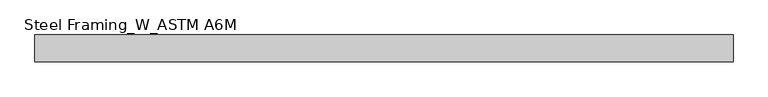
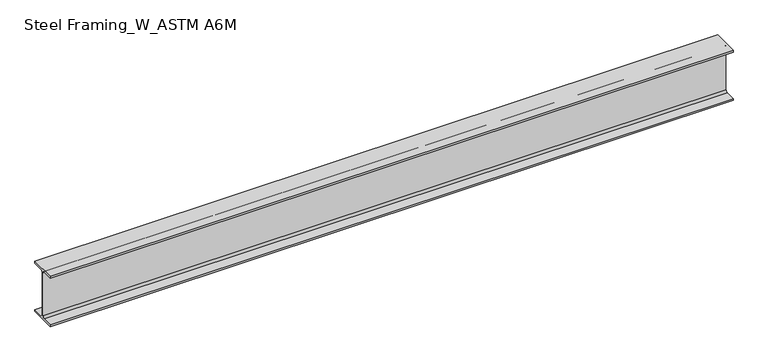
"""IFC4 building model written with IfcOpenShell, lengths in millimetres: beam geometry, Steel Framing_W_ASTM A6M : H_SB_AR_S02_W200x22.5_J1."""

import ifcopenshell
import ifcopenshell.guid

model = None  # the IFC model being written
_history = None  # IfcOwnerHistory: only IFC2X3 demands one
_inside = {}  # id of a spatial element -> (the spatial element, [elements in it])
_under = {}  # id of a project, library or spatial element -> (it, [spatial elements below it])
_declared = {}  # id of a project -> (the project, [libraries it declares])
_typed = {}  # id of a type object -> (the type object, [elements of that type])
_made_of = {}  # id of a material, layer set ... -> (it, [elements and type objects made of it])


def new_model(schema):
    """Start an empty IFC model of exactly this schema.

    Asked for "IFC4X3", IfcOpenShell would pick the latest addendum, in which some entities
    have other attributes; the version numbers below select the first issue.
    IFC2X3 requires an IfcOwnerHistory on every rooted entity: one is made here for all.
    """
    global model, _history
    if schema == "IFC4X3":
        model = ifcopenshell.file(schema_version=(4, 3, 0, 0))
    else:
        model = ifcopenshell.file(schema=schema)
    _inside.clear()
    _under.clear()
    _declared.clear()
    _typed.clear()
    _made_of.clear()
    _history = None
    if model.schema == "IFC2X3":
        org = make("IfcOrganization", Name="unknown")
        user = make(
            "IfcPersonAndOrganization",
            ThePerson=make("IfcPerson", FamilyName="unknown"),
            TheOrganization=org,
        )
        app = make(
            "IfcApplication",
            ApplicationDeveloper=org,
            Version="unknown",
            ApplicationFullName="unknown",
            ApplicationIdentifier="unknown",
        )
        _history = make(
            "IfcOwnerHistory",
            OwningUser=user,
            OwningApplication=app,
            ChangeAction="ADDED",
            CreationDate=0,
        )
    return model


def make(cls, **values):
    """One entity of the class cls with the attributes given. An attribute that is None is left unset."""
    return model.create_entity(
        cls, **{name: value for name, value in values.items() if value is not None}
    )


def rooted(cls, **values):
    """An entity with a GlobalId (a new one), such as an element, a storey or a relation."""
    return make(cls, GlobalId=ifcopenshell.guid.new(), OwnerHistory=_history, **values)


def si_unit(unit_type, name, prefix=None):
    """IfcSIUnit, for example si_unit("LENGTHUNIT", "METRE", prefix="MILLI")."""
    return make("IfcSIUnit", UnitType=unit_type, Prefix=prefix, Name=name)


def assignment(units):
    """IfcUnitAssignment: the units of a project."""
    return None if units is None else make("IfcUnitAssignment", Units=units)


def point(xyz):
    """IfcCartesianPoint."""
    return None if xyz is None else make("IfcCartesianPoint", Coordinates=xyz)


def direction(xyz):
    """IfcDirection."""
    return None if xyz is None else make("IfcDirection", DirectionRatios=xyz)


def frame(location, z_axis=None, x_axis=None):
    """IfcAxis2Placement3D, a coordinate frame: its origin and axes. An axis left out is left unset."""
    return make(
        "IfcAxis2Placement3D",
        Location=point(location),
        Axis=direction(z_axis),
        RefDirection=direction(x_axis),
    )


def frame_2d(location, x_axis=None):
    """IfcAxis2Placement2D, a coordinate frame in the plane: its origin and x axis."""
    return make(
        "IfcAxis2Placement2D", Location=point(location), RefDirection=direction(x_axis)
    )


def origin():
    """The frame at (0, 0, 0) with its axes left unset."""
    return frame((0.0, 0.0, 0.0))


def place(relative_to, where):
    """IfcLocalPlacement: puts the frame where relative to a parent placement (None: the world)."""
    return make(
        "IfcLocalPlacement", PlacementRelTo=relative_to, RelativePlacement=where
    )


def context(
    kind, dimensions, precision=None, world=None, true_north=None, identifier=None
):
    """IfcGeometricRepresentationContext, for example the 3D "Model" context."""
    return make(
        "IfcGeometricRepresentationContext",
        ContextIdentifier=identifier,
        ContextType=kind,
        CoordinateSpaceDimension=dimensions,
        Precision=precision,
        WorldCoordinateSystem=world,
        TrueNorth=true_north,
    )


def project(units=None, contexts=None):
    """IfcProject with its units and contexts."""
    return rooted(
        "IfcProject",
        Name="project",
        RepresentationContexts=contexts,
        UnitsInContext=assignment(units),
    )


def spatial(cls, under=None, at=None, **own):
    """A site, building, storey or space (cls), placed at a placement, below another one or the project."""
    s = rooted(cls, ObjectPlacement=at, **own)
    if under is not None:
        _under.setdefault(under.id(), (under, []))[1].append(s)
    return s


def polyline(points):
    """IfcPolyline through the points."""
    return make("IfcPolyline", Points=[point(p) for p in points])


def circle_curve(where, radius):
    """IfcCircle in the frame where."""
    return make("IfcCircle", Position=where, Radius=radius)


def trimmed(basis, trim1, trim2, sense, master):
    """IfcTrimmedCurve: the piece of a basis curve between two trims."""
    return make(
        "IfcTrimmedCurve",
        BasisCurve=basis,
        Trim1=trim1,
        Trim2=trim2,
        SenseAgreement=sense,
        MasterRepresentation=master,
    )


def segment(curve, same_sense, transition):
    """IfcCompositeCurveSegment."""
    return make(
        "IfcCompositeCurveSegment",
        Transition=transition,
        SameSense=same_sense,
        ParentCurve=curve,
    )


def composite_curve(segments, self_intersect=None):
    """IfcCompositeCurve: segments joined end to end."""
    return make("IfcCompositeCurve", Segments=segments, SelfIntersect=self_intersect)


def outline(outer, holes=None, kind="AREA"):
    """IfcArbitraryClosedProfileDef: a profile drawn as a closed curve; with holes, ...WithVoids."""
    if holes is None:
        return make("IfcArbitraryClosedProfileDef", ProfileType=kind, OuterCurve=outer)
    return make(
        "IfcArbitraryProfileDefWithVoids",
        ProfileType=kind,
        OuterCurve=outer,
        InnerCurves=holes,
    )


def extrude(swept, where, along, depth):
    """IfcExtrudedAreaSolid: the profile swept, set in the frame where, extruded along a direction by depth."""
    return make(
        "IfcExtrudedAreaSolid",
        SweptArea=swept,
        Position=where,
        ExtrudedDirection=direction(along),
        Depth=depth,
    )


def shape(context_of_items, identifier, shape_type, items):
    """IfcShapeRepresentation: the items that make up one representation, for example the "Body"."""
    return make(
        "IfcShapeRepresentation",
        ContextOfItems=context_of_items,
        RepresentationIdentifier=identifier,
        RepresentationType=shape_type,
        Items=items,
    )


def source(mapping_origin, context_of_items, identifier, shape_type, items):
    """IfcRepresentationMap: a shape defined once, which mapped items show again and again."""
    return make(
        "IfcRepresentationMap",
        MappingOrigin=mapping_origin,
        MappedRepresentation=shape(context_of_items, identifier, shape_type, items),
    )


def transform(
    local_origin,
    x_axis=None,
    y_axis=None,
    z_axis=None,
    scale=None,
    scale2=None,
    scale3=None,
    uniform=True,
):
    """IfcCartesianTransformationOperator3D, or its non-uniform kind. x_axis, y_axis, z_axis: its Axis1, 2, 3."""
    if uniform:
        return make(
            "IfcCartesianTransformationOperator3D",
            Axis1=direction(x_axis),
            Axis2=direction(y_axis),
            LocalOrigin=point(local_origin),
            Scale=scale,
            Axis3=direction(z_axis),
        )
    return make(
        "IfcCartesianTransformationOperator3DnonUniform",
        Axis1=direction(x_axis),
        Axis2=direction(y_axis),
        LocalOrigin=point(local_origin),
        Scale=scale,
        Axis3=direction(z_axis),
        Scale2=scale2,
        Scale3=scale3,
    )


def mapped(mapping_source, mapping_target):
    """IfcMappedItem: shows the shape of a source again, moved by a transform."""
    return make(
        "IfcMappedItem", MappingSource=mapping_source, MappingTarget=mapping_target
    )


def made_of(thing, what):
    """Note that an element or type object is made of a material, layer set ...; save() writes the relation."""
    if what is not None:
        _made_of.setdefault(what.id(), (what, []))[1].append(thing)
    return thing


def element(
    cls,
    number,
    at=None,
    inside=None,
    cuts=None,
    type_object=None,
    material=None,
    context=None,
    identifier="Body",
    shape_type=None,
    held_by="IfcProductDefinitionShape",
    body=None,
    shapes=None,
    **own,
):
    """One element of the class cls, such as IfcWall. Its Tag is "e" and its number.

    at: its placement. inside: the storey or other place that contains it. cuts: it is an
    opening in that element (IfcRelVoidsElement). A single representation is given by context,
    identifier, shape_type and body (its items); several are given by shapes. held_by: the class
    of the entity that holds the representations. save() writes the other relations.
    """
    e = rooted(cls, Tag="e%d" % number, ObjectPlacement=at, **own)
    if body is not None:
        shapes = [shape(context, identifier, shape_type, body)]
    if shapes is not None:
        e.Representation = make(held_by, Representations=shapes)
    if inside is not None:
        _inside.setdefault(inside.id(), (inside, []))[1].append(e)
    if cuts is not None:
        rooted(
            "IfcRelVoidsElement", RelatingBuildingElement=cuts, RelatedOpeningElement=e
        )
    if type_object is not None:
        _typed.setdefault(type_object.id(), (type_object, []))[1].append(e)
    return made_of(e, material)


def aggregate(whole, parts):
    """IfcRelAggregates: a whole, such as a stair, and the parts it consists of."""
    return rooted("IfcRelAggregates", RelatingObject=whole, RelatedObjects=parts)


def save(model, path):
    """Write the relations noted so far, then the file.

    IfcRelAggregates (storeys below a building ...), IfcRelContainedInSpatialStructure (elements
    in a storey), IfcRelDefinesByType, IfcRelAssociatesMaterial and IfcRelDeclares: one each for
    every whole, place, type object, material and project.
    """
    for whole, parts in _under.values():
        aggregate(whole, parts)
    for where, things in _inside.values():
        rooted(
            "IfcRelContainedInSpatialStructure",
            RelatedElements=things,
            RelatingStructure=where,
        )
    for kind, things in _typed.values():
        rooted("IfcRelDefinesByType", RelatedObjects=things, RelatingType=kind)
    for what, things in _made_of.values():
        rooted("IfcRelAssociatesMaterial", RelatedObjects=things, RelatingMaterial=what)
    for by, libraries in _declared.values():
        rooted("IfcRelDeclares", RelatingContext=by, RelatedDefinitions=libraries)
    model.write(path)


def steel_framing_w_astm_a6m_d2b621d1(model_context):
    return source(origin(), model_context, "Body", "SweptSolid", [
        extrude(outline(composite_curve([segment(polyline([(51.0, -95.0), (51.0, -103.0), (-51.0, -103.0), (-51.0, -95.0), (-10.71, -95.0)]), True, "CONTINUOUS"), segment(trimmed(circle_curve(frame_2d((-10.71, -87.4)), 7.6), [point((-10.71, -95.0))], [point((-3.11, -87.4))], True, "CARTESIAN"), True, "CONTINUOUS"), segment(polyline([(-3.11, -87.4), (-3.11, 87.4)]), True, "CONTINUOUS"), segment(trimmed(circle_curve(frame_2d((-10.71, 87.4)), 7.6), [point((-3.11, 87.4))], [point((-10.71, 95.0))], True, "CARTESIAN"), True, "CONTINUOUS"), segment(polyline([(-10.71, 95.0), (-51.0, 95.0), (-51.0, 103.0), (51.0, 103.0), (51.0, 95.0), (10.71, 95.0)]), True, "CONTINUOUS"), segment(trimmed(circle_curve(frame_2d((10.71, 87.4)), 7.6), [point((10.71, 95.0))], [point((3.11, 87.4))], True, "CARTESIAN"), True, "CONTINUOUS"), segment(polyline([(3.11, 87.4), (3.11, -87.4)]), True, "CONTINUOUS"), segment(trimmed(circle_curve(frame_2d((10.71, -87.4)), 7.6), [point((3.11, -87.4))], [point((10.71, -95.0))], True, "CARTESIAN"), True, "CONTINUOUS"), segment(polyline([(10.71, -95.0), (51.0, -95.0)]), True, "CONTINUOUS")], self_intersect=False)), frame((-1319.7, 0.0, 0.0), z_axis=(1.0, 0.0, 0.0), x_axis=(0.0, 1.0, 0.0)), (0.0, 0.0, 1.0), 2639.4),
    ])


if __name__ == "__main__":
    model = new_model("IFC4")
    model_context = context("Model", 3, world=origin())
    ifc_project = project(units=[si_unit("LENGTHUNIT", "METRE", prefix="MILLI")], contexts=[model_context])
    site = spatial("IfcSite", under=ifc_project)
    building = spatial("IfcBuilding", under=site)
    placement = place(None, origin())
    steel_framing_w_astm_a6m_shape = steel_framing_w_astm_a6m_d2b621d1(model_context)
    element("IfcBeam", 1, ObjectType="Steel Framing_W_ASTM A6M : H_SB_AR_S02_W200x22.5_J1", at=placement, inside=building, context=model_context, shape_type="MappedRepresentation", body=[
        mapped(steel_framing_w_astm_a6m_shape, transform((0.0, 0.0, 0.0), x_axis=(1.0, 0.0, 0.0), y_axis=(0.0, 1.0, 0.0), z_axis=(0.0, 0.0, 1.0))),
    ])
    save(model, "model.ifc")

# Revit data of these elements
# Type "Steel Framing_W_ASTM A6M : H_SB_AR_S02_W200x22.5_J1"
#   Section Name Key = "W8x15"
#   Width = 10.2 cm
#   Web Thickness = 0.622 cm
#   Web Fillet = 0.76 cm
#   Warping Constant = 13900.0 cm⁶
#   Torsional Moment of Inertia = 5.70 cm⁴
#   Section Area = 28.6 cm²
#   Plastic Modulus weak axis = 43.8 cm³
#   Plastic Modulus strong axis = 223.0 cm³
#   Perimeter = 0.795 m²/m
#   Nominal Weight = 22.50 kgf/m
#   Moment of Inertia weak axis = 142.00 cm⁴
#   Moment of Inertia strong axis = 2000.00 cm⁴
#   Height = 20.6 cm
#   Flange Thickness = 0.8 cm
#   Elastic Modulus weak axis = 27.9 cm³
#   Elastic Modulus strong axis = 193.0 cm³
#   Centroid Vertical = 10.3 cm
#   Centroid Horizontal = 5.1 cm
#   Length [instance default] = 1500 mm
#   Structural Material [instance default] = Steel, 45-345
#   Bolt Spacing = 0
#   Assembly Code = ""
# Element 1 (IfcBeam, "Steel Framing_W_ASTM A6M : H_SB_AR_S02_W200x22.5_J1")
#   Materials on its faces: "Steel, 45-345"
# Materials
#   "Steel, 45-345": class "Metal", colour RGB 189 187 185, transparency 0, Description = "Steel 345 MPa", Cost = 0
